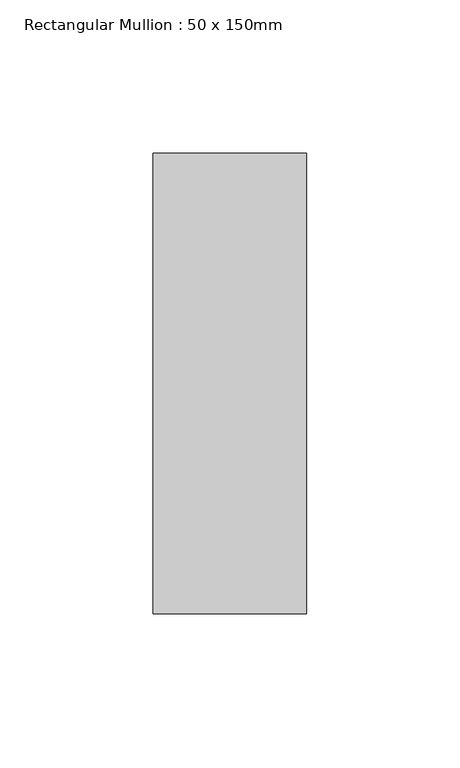
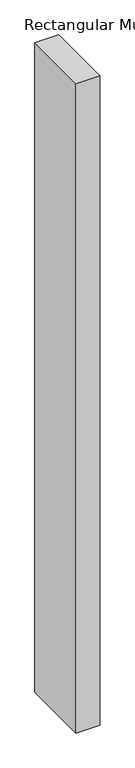
"""IFC4 building model written with IfcOpenShell, lengths in millimetres: member geometry, Rectangular Mullion : 50 x 150mm."""

from ifc_helpers import new_model, si_unit, frame, origin, place, context, project, spatial, polyline, outline, extrude, source, transform, mapped, element, save


def rectangular_mullion_50_x_150mm_e3a7335b(model_context):
    return source(origin(), model_context, "Body", "SweptSolid", [
        extrude(outline(polyline([(0.0, 75.0), (0.0, -75.0), (-50.0, -75.0), (-50.0, 75.0), (0.0, 75.0)])), frame((0.0, 0.0, -1449.9999998), z_axis=(0.0, 0.0, 1.0), x_axis=(1.0, 0.0, 0.0)), (0.0, 0.0, 1.0), 1449.9999998),
    ])


if __name__ == "__main__":
    model = new_model("IFC4")
    model_context = context("Model", 3, world=origin())
    ifc_project = project(units=[si_unit("LENGTHUNIT", "METRE", prefix="MILLI")], contexts=[model_context])
    site = spatial("IfcSite", under=ifc_project)
    building = spatial("IfcBuilding", under=site)
    placement = place(None, origin())
    rectangular_mullion_50_x_150mm_shape = rectangular_mullion_50_x_150mm_e3a7335b(model_context)
    element("IfcMember", 1, ObjectType="Rectangular Mullion : 50 x 150mm", at=placement, inside=building, context=model_context, shape_type="MappedRepresentation", body=[
        mapped(rectangular_mullion_50_x_150mm_shape, transform((0.0, 0.0, 0.0), x_axis=(1.0, 0.0, 0.0), y_axis=(0.0, 1.0, 0.0), z_axis=(0.0, 0.0, 1.0))),
    ])
    save(model, "model.ifc")

# Revit data of these elements
# Type "Rectangular Mullion : 50 x 150mm"
#   built-in parameter 1007304 = 0.492126 (stored number, unit not read)
#   built-in parameter 1007301 = 0.082021 (stored number, unit not read)
#   built-in parameter 1007300 = 0.082021 (stored number, unit not read)
# Element 1 (IfcMember, "Rectangular Mullion : 50 x 150mm")
#   Materials on its faces: "Aluminium"
# Materials
#   "Aluminium": class "Metal", colour RGB 247 247 247, transparency 0, Description = "Aluminium 6061", Cost = 0
